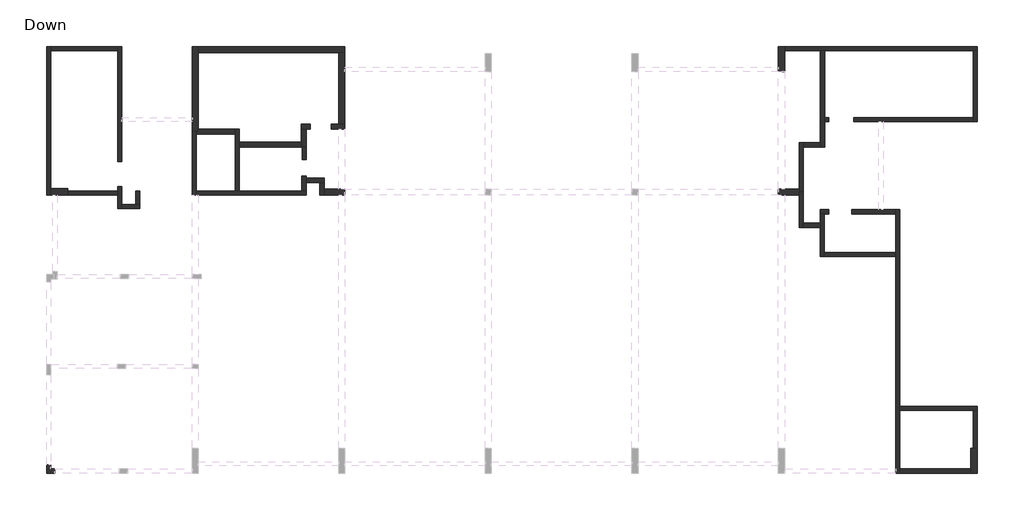
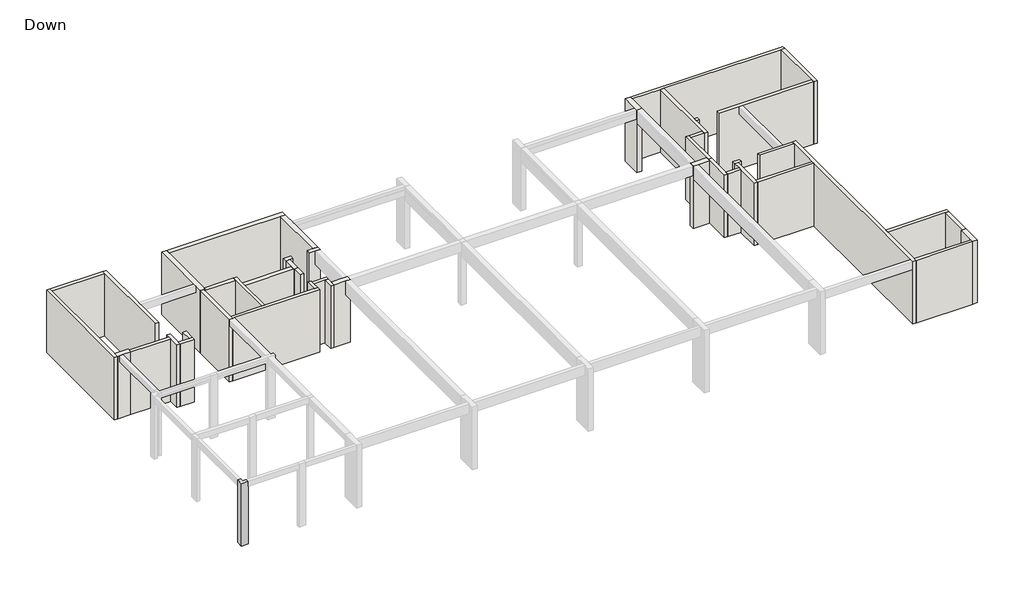
# One storey, part 1 of 2: 44 walls, 1 column.
# Revit data of these elements (continued)
# Element 36 (IfcWall, "25") (continued)
#   SOFiSTiK_AMG_Scheduled = yes
#   SOFiSTiK_AMG_Adjusted = yes
#   Phase Created = New Construction
#   Base Constraint = Down
#   Top Constraint = Typical Floor
#   Materials on its faces: "Concrete"
# Element 37 (IfcWall, "25")
#   Comments = ""
#   Mark = "W44"
#   SOFiSTiK_EdgeZones = "W44"
#   SOFiSTiK_AMG_Comments = ""
#   Top Offset = 0 cm
#   Base Offset = 0 cm
#   Unconnected Height = 400 cm
#   wall height = 400 cm
#   SOFiSTiK_AMG_Scheduled = yes
#   SOFiSTiK_AMG_Adjusted = yes
#   Phase Created = New Construction
#   Base Constraint = Down
#   Top Constraint = Typical Floor
#   Materials on its faces: "Concrete"
# Element 38 (IfcWall, "30")
#   Comments = ""
#   Mark = "W32"
#   SOFiSTiK_EdgeZones = "W32"
#   SOFiSTiK_AMG_Comments = ""
#   Top Offset = 0 cm
#   Base Offset = 0 cm
#   Unconnected Height = 400 cm
#   wall height = 400 cm
#   SOFiSTiK_AMG_Scheduled = yes
#   SOFiSTiK_AMG_Adjusted = yes
#   Phase Created = New Construction
#   Base Constraint = Down
#   Top Constraint = Typical Floor
#   Materials on its faces: "Concrete"
# Element 39 (IfcWall, "30")
#   Comments = ""
#   Mark = "W33"
#   SOFiSTiK_EdgeZones = "W33"
#   SOFiSTiK_AMG_Comments = ""
#   Top Offset = 0 cm
#   Base Offset = 0 cm
#   Unconnected Height = 400 cm
#   wall height = 400 cm
#   SOFiSTiK_AMG_Scheduled = yes
#   SOFiSTiK_AMG_Adjusted = yes
#   Phase Created = New Construction
#   Base Constraint = Down
#   Top Constraint = Typical Floor
#   Materials on its faces: "Concrete"
# Element 40 (IfcWall, "30")
#   Comments = ""
#   Mark = "W34"
#   SOFiSTiK_EdgeZones = "W34"
#   SOFiSTiK_AMG_Comments = ""
#   Top Offset = 0 cm
#   Base Offset = 0 cm
#   Unconnected Height = 400 cm
#   wall height = 400 cm
#   SOFiSTiK_AMG_Scheduled = yes
#   SOFiSTiK_AMG_Adjusted = yes
#   Phase Created = New Construction
#   Base Constraint = Down
#   Top Constraint = Typical Floor
#   Materials on its faces: "Concrete"
# Element 41 (IfcWall, "30")
#   Comments = ""
#   Mark = "W35"
#   SOFiSTiK_EdgeZones = "W35"
#   SOFiSTiK_AMG_Comments = ""
#   Top Offset = 0 cm
#   Base Offset = 0 cm
#   Unconnected Height = 400 cm
#   wall height = 400 cm
#   SOFiSTiK_AMG_Scheduled = yes
#   SOFiSTiK_AMG_Adjusted = yes
#   Phase Created = New Construction
#   Base Constraint = Down
#   Top Constraint = Typical Floor
#   Materials on its faces: "Concrete"
# Element 42 (IfcWall, "30")
#   Comments = ""
#   Mark = "W36"
#   SOFiSTiK_EdgeZones = "W36"
#   SOFiSTiK_AMG_Comments = ""
#   Top Offset = 0 cm
#   Base Offset = 0 cm
#   Unconnected Height = 400 cm
#   wall height = 400 cm
#   SOFiSTiK_AMG_Scheduled = yes
#   SOFiSTiK_AMG_Adjusted = yes
#   Phase Created = New Construction
#   Base Constraint = Down
#   Top Constraint = Typical Floor
#   Materials on its faces: "Concrete"
# Element 43 (IfcWall, "30")
#   Comments = ""
#   Mark = "W37"
#   SOFiSTiK_EdgeZones = "W37"
#   SOFiSTiK_AMG_Comments = ""
#   Top Offset = 0 cm
#   Base Offset = 0 cm
#   Unconnected Height = 400 cm
#   wall height = 400 cm
#   SOFiSTiK_AMG_Scheduled = yes
#   SOFiSTiK_AMG_Adjusted = yes
#   Phase Created = New Construction
#   Base Constraint = Down
#   Top Constraint = Typical Floor
#   Materials on its faces: "Concrete"
# Element 44 (IfcWall, "30")
#   Comments = ""
#   Mark = "W38"
#   SOFiSTiK_EdgeZones = "W38"
#   SOFiSTiK_AMG_Comments = ""
#   Top Offset = 0 cm
#   Base Offset = 0 cm
#   Unconnected Height = 400 cm
#   wall height = 400 cm
#   SOFiSTiK_AMG_Scheduled = yes
#   SOFiSTiK_AMG_Adjusted = yes
#   Phase Created = New Construction
#   Base Constraint = Down
#   Top Constraint = Typical Floor
#   Materials on its faces: "Concrete"
# Element 45 (IfcWall, "30")
#   Comments = ""
#   Mark = "W39"
#   SOFiSTiK_EdgeZones = "W39"
#   SOFiSTiK_AMG_Comments = ""
#   Top Offset = 0 cm
#   Base Offset = 0 cm
#   Unconnected Height = 400 cm
#   wall height = 400 cm
#   SOFiSTiK_AMG_Scheduled = yes
#   SOFiSTiK_AMG_Adjusted = yes
#   Phase Created = New Construction
#   Base Constraint = Down
#   Top Constraint = Typical Floor
#   Materials on its faces: "Concrete"
# Materials
#   "Concrete, Cast-in-Place gray": class "Concrete", colour RGB 192 192 192, transparency 0, Description = "Cast-in-place concrete", Cost = 0
#   "Concrete": class "Concrete", colour RGB 192 192 192, transparency 0, Keynote = "01000", Description = "Cast-in-place concrete", Cost = 0
